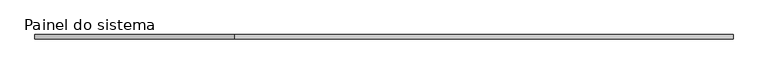
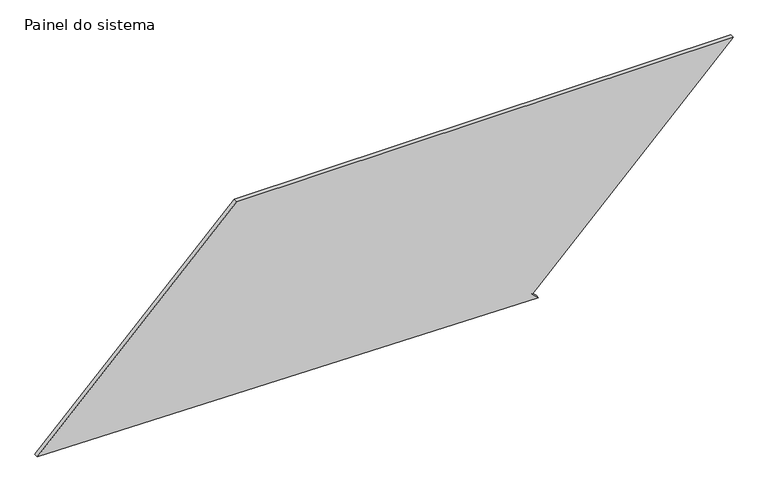
"""IFC4 building model written with IfcOpenShell, lengths in millimetres: plate geometry, Painel do sistema : Envidraçado."""

from ifc_helpers import new_model, si_unit, frame, origin, place, context, project, spatial, polyline, outline, extrude, source, transform, mapped, element, save


def painel_do_sistema_6d478be6(model_context):
    return source(origin(), model_context, "Body", "SweptSolid", [
        extrude(outline(polyline([(0.0, 899.002678), (35.3105361, 863.6025926), (1215.435386, 2040.7421586), (1215.435386, -871.4758131), (43.2037234, -2040.7421586), (0.0, 899.002678)])), frame((0.0, 24.5, 0.0), z_axis=(0.0, 1.0, 0.0), x_axis=(0.0, 0.0, 1.0)), (0.0, 0.0, 1.0), 25.0),
    ])


if __name__ == "__main__":
    model = new_model("IFC4")
    model_context = context("Model", 3, world=origin())
    ifc_project = project(units=[si_unit("LENGTHUNIT", "METRE", prefix="MILLI")], contexts=[model_context])
    site = spatial("IfcSite", under=ifc_project)
    building = spatial("IfcBuilding", under=site)
    placement = place(None, origin())
    painel_do_sistema_shape = painel_do_sistema_6d478be6(model_context)
    element("IfcPlate", 1, ObjectType="Painel do sistema : Envidraçado", at=placement, inside=building, context=model_context, shape_type="MappedRepresentation", body=[
        mapped(painel_do_sistema_shape, transform((0.0, 0.0, 0.0), x_axis=(1.0, 0.0, 0.0), y_axis=(0.0, 1.0, 0.0), z_axis=(0.0, 0.0, 1.0))),
    ])
    save(model, "model.ifc")

# Revit data of these elements
# Type "Painel do sistema : Envidraçado"
#   Construction Type Id = "GSP4R"
#   Analytic Construction = "Vidraça única Pilkington 1/8 pol"
#   Visual Light Transmittance = 0.9
#   Solar Heat Gain Coefficient = 0.86
#   Heat Transfer Coefficient (U) = 6.7069 W/(m²·K)
# Element 1 (IfcPlate, "Painel do sistema : Envidraçado")
#   Materials on its faces: "Vidro"
# Materials
#   "Vidro": class "Vidro", colour RGB 0 128 192, transparency 0.9, Description = "Vidro de sílica", Cost = 0
